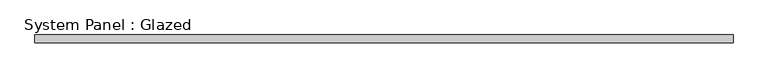
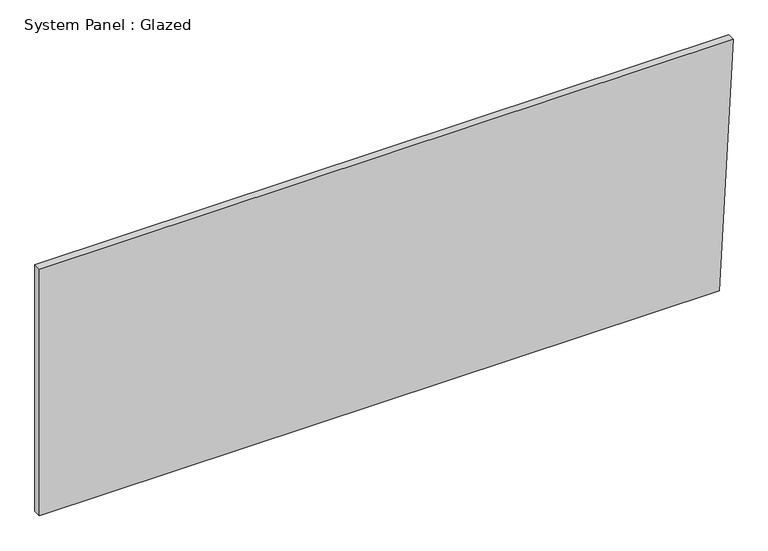
"""IFC4 building model written with IfcOpenShell, lengths in millimetres: plate geometry, System Panel : Glazed."""

from ifc_helpers import new_model, si_unit, frame, origin, place, context, project, spatial, polyline, outline, extrude, source, transform, mapped, element, save


def system_panel_glazed_5a6bcccf(model_context):
    return source(origin(), model_context, "Body", "SweptSolid", [
        extrude(outline(polyline([(0.0, -1151.5076076), (0.0, 1106.180401), (866.081558, 1151.5076076), (866.081558, -1151.5076076), (0.0, -1151.5076076)])), frame((0.0, -44.45, 0.0), z_axis=(0.0, 1.0, 0.0), x_axis=(0.0, 0.0, 1.0)), (0.0, 0.0, 1.0), 25.4),
    ])


if __name__ == "__main__":
    model = new_model("IFC4")
    model_context = context("Model", 3, world=origin())
    ifc_project = project(units=[si_unit("LENGTHUNIT", "METRE", prefix="MILLI")], contexts=[model_context])
    site = spatial("IfcSite", under=ifc_project)
    building = spatial("IfcBuilding", under=site)
    placement = place(None, origin())
    system_panel_glazed_shape = system_panel_glazed_5a6bcccf(model_context)
    element("IfcPlate", 1, ObjectType="System Panel : Glazed", at=placement, inside=building, context=model_context, shape_type="MappedRepresentation", body=[
        mapped(system_panel_glazed_shape, transform((0.0, 0.0, 0.0), x_axis=(1.0, 0.0, 0.0), y_axis=(0.0, 1.0, 0.0), z_axis=(0.0, 0.0, 1.0))),
    ])
    save(model, "model.ifc")

# Revit data of these elements
# Type "System Panel : Glazed"
#   Construction Type Id = "GSP4R"
#   Analytic Construction = "1/8 in Pilkington single glazing"
#   Visual Light Transmittance = 0.9
#   Solar Heat Gain Coefficient = 0.86
#   Heat Transfer Coefficient (U) = 1.18115 BTU/(h·ft²·°F)
#   Define Thermal Properties by = 1
# Element 1 (IfcPlate, "System Panel : Glazed")
#   Materials on its faces: "Glass"
# Materials
#   "Glass": class "Glass", colour RGB 0 128 192, transparency 0.75, Description = "Soda Lime Glass", Cost = 0
